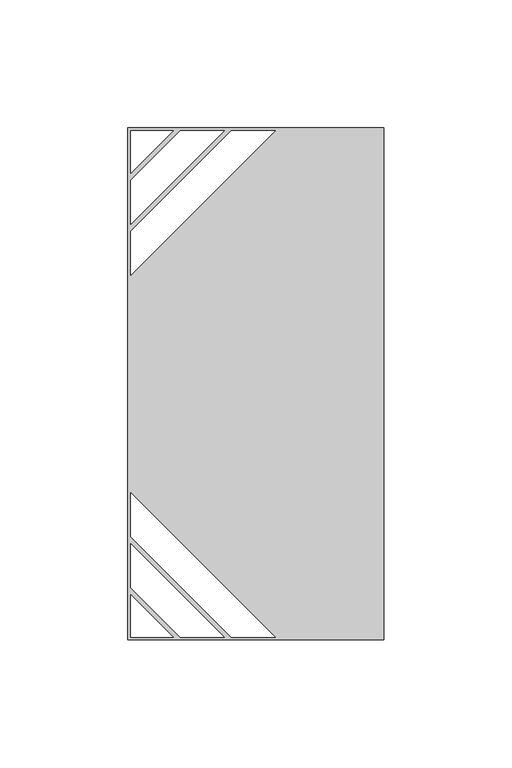
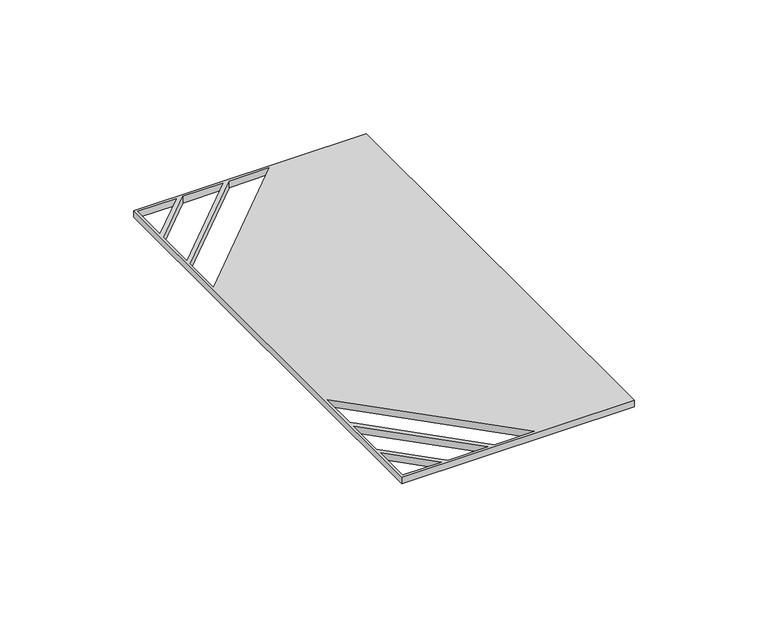
"""IFC4 building model written with IfcOpenShell, lengths in millimetres: proxy geometry, TSP Heated Pool and Jacuzzi Supply only : TSP Heated Pool and Jacuzzi Supply only."""

from ifc_helpers import new_model, si_unit, origin, origin_with_axes, place, context, project, spatial, polyline, outline, extrude, source, transform, mapped, element, save


def electrical_fixtures_068ecc0e(model_context):
    return source(origin(), model_context, "Body", "SweptSolid", [
        extrude(outline(polyline([(-100.0, 100.0), (0.0, 100.0), (0.0, -100.0), (-100.0, -100.0), (-100.0, 100.0)]), holes=[polyline([(-59.5857864, 99.0), (-99.0, 59.5857864), (-99.0, 42.4142136), (-42.4142136, 99.0), (-59.5857864, 99.0)]), polyline([(-99.0, 82.4142136), (-82.4142136, 99.0), (-99.0, 99.0), (-99.0, 82.4142136)]), polyline([(-99.0, 79.5857864), (-99.0, 62.4142136), (-62.4142136, 99.0), (-79.5857864, 99.0), (-99.0, 79.5857864)]), polyline([(-59.5857864, -99.0), (-42.4142136, -99.0), (-99.0, -42.4142136), (-99.0, -59.5857864), (-59.5857864, -99.0)]), polyline([(-99.0, -82.4142136), (-99.0, -99.0), (-82.4142136, -99.0), (-99.0, -82.4142136)]), polyline([(-99.0, -79.5857864), (-79.5857864, -99.0), (-62.4142136, -99.0), (-99.0, -62.4142136), (-99.0, -79.5857864)])]), origin_with_axes(), (0.0, 0.0, 1.0), 3.0),
    ])


if __name__ == "__main__":
    model = new_model("IFC4")
    model_context = context("Model", 3, world=origin())
    ifc_project = project(units=[si_unit("LENGTHUNIT", "METRE", prefix="MILLI")], contexts=[model_context])
    site = spatial("IfcSite", under=ifc_project)
    building = spatial("IfcBuilding", under=site)
    placement = place(None, origin())
    electrical_fixtures_shape = electrical_fixtures_068ecc0e(model_context)
    element("IfcBuildingElementProxy", 1, Name="TSP Heated Pool and Jacuzzi Supply only : TSP Heated Pool and Jacuzzi Supply only", ObjectType="TSP Heated Pool and Jacuzzi Supply only : TSP Heated Pool and Jacuzzi Supply only", at=placement, inside=building, context=model_context, shape_type="MappedRepresentation", body=[
        mapped(electrical_fixtures_shape, transform((0.0, 0.0, 0.0), x_axis=(1.0, 0.0, 0.0), y_axis=(0.0, 1.0, 0.0), z_axis=(0.0, 0.0, 1.0))),
    ])
    save(model, "model.ifc")

# Revit data of these elements
# Type "TSP Heated Pool and Jacuzzi Supply only : TSP Heated Pool and Jacuzzi Supply only"
#   Model = "TSP_ELECSPJZHOT"
#   Default Elevation = 0
# Element 1 (IfcBuildingElementProxy, "TSP Heated Pool and Jacuzzi Supply only : TSP Heated Pool and Jacuzzi Supply only")
#   Materials on its faces: "Plastic, Opaque Black"
# Materials
#   "Plastic, Opaque Black": class "Plastic", colour RGB 0 0 0, transparency 0.7, Description = "Plastic, generic, opaque black", Cost = 0
